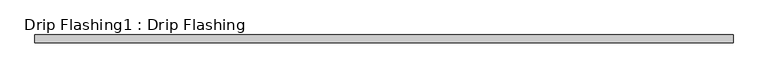
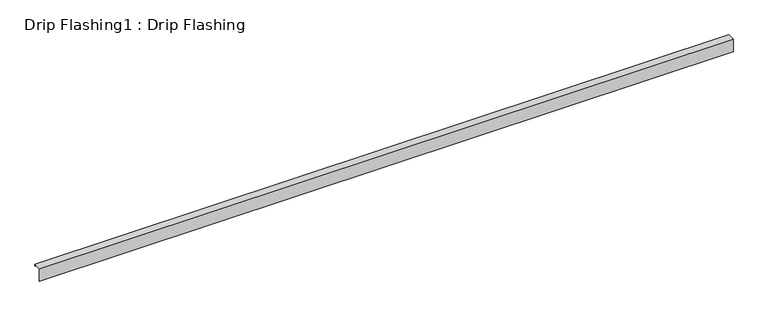
"""IFC4 building model written with IfcOpenShell, lengths in millimetres: proxy geometry, Drip Flashing1 : Drip Flashing."""

from ifc_helpers import new_model, si_unit, frame, origin, place, context, project, spatial, polyline, outline, extrude, source, transform, mapped, element, save


def drip_flashing1_drip_flashing_f6117538(model_context):
    return source(origin(), model_context, "Body", "SweptSolid", [
        extrude(outline(polyline([(9742.6949545, 37596.6323438), (9742.6949545, 37559.8023438), (9741.4249545, 37559.8023438), (9741.4249545, 37597.9023438), (9763.6499545, 37597.9023438), (9763.6499545, 37593.1525438), (9760.6474981, 37593.1525438), (9760.6474981, 37594.4225437), (9762.3799545, 37594.4225437), (9762.3799545, 37596.6323438), (9742.6949545, 37596.6323438)])), frame((-9232.0719278, 0.0, 0.0), z_axis=(1.0, 0.0, 0.0), x_axis=(0.0, 1.0, 0.0)), (0.0, 0.0, 1.0), 1999.85),
    ])


if __name__ == "__main__":
    model = new_model("IFC4")
    model_context = context("Model", 3, world=origin())
    ifc_project = project(units=[si_unit("LENGTHUNIT", "METRE", prefix="MILLI")], contexts=[model_context])
    site = spatial("IfcSite", under=ifc_project)
    building = spatial("IfcBuilding", under=site)
    placement = place(None, origin())
    drip_flashing1_drip_flashing_shape = drip_flashing1_drip_flashing_f6117538(model_context)
    element("IfcBuildingElementProxy", 1, Name="Drip Flashing1 : Drip Flashing", ObjectType="Drip Flashing1 : Drip Flashing", at=placement, inside=building, context=model_context, shape_type="MappedRepresentation", body=[
        mapped(drip_flashing1_drip_flashing_shape, transform((0.0, 0.0, 0.0), x_axis=(1.0, 0.0, 0.0), y_axis=(0.0, 1.0, 0.0), z_axis=(0.0, 0.0, 1.0))),
    ])
    save(model, "model.ifc")

# Revit data of these elements
# Type "Drip Flashing1 : Drip Flashing"
#   NameOverride = "Drip Flashing"
# Element 1 (IfcBuildingElementProxy, "Drip Flashing1 : Drip Flashing")
#   Materials on its faces: "COPPER STUCCO J BEAD"
# Materials
#   "COPPER STUCCO J BEAD": class "Unassigned", colour RGB 251 232 155, transparency 0, Cost = 0
